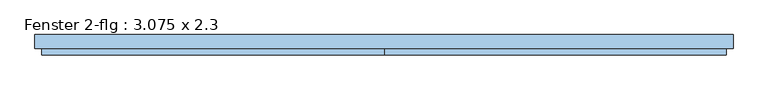
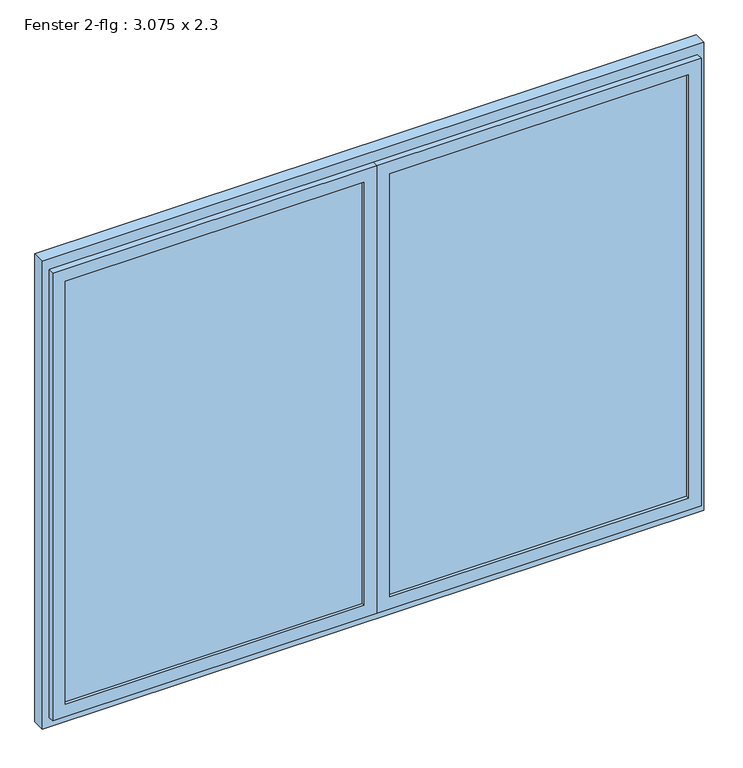
"""IFC4 building model written with IfcOpenShell, lengths in millimetres: window geometry, Fenster 2-flg : 3.075 x 2.3."""

from ifc_helpers import new_model, si_unit, frame, origin, place, context, project, spatial, polyline, outline, extrude, faceted_brep, source, transform, mapped, element, save


def fenster_2_flg_3_075_x_2_3_a01fdd74(model_context):
    return source(origin(), model_context, "Body", "SolidModel", [
        extrude(outline(polyline([(30.0, -30.0), (-30.0, -30.0), (-30.0, 30.0), (30.0, 30.0), (30.0, -30.0)])), frame((0.0, 0.0, 1080.0), z_axis=(0.0, 0.0, 1.0), x_axis=(1.0, 0.0, 0.0)), (0.0, 0.0, 1.0), 2140.0),
        extrude(outline(polyline([(3300.0, -1537.5), (1000.0, -1537.5), (1000.0, 1537.5), (3300.0, 1537.5), (3300.0, -1537.5)]), holes=[polyline([(3220.0, -1477.5), (3220.0, 1477.5), (1080.0, 1477.5), (1080.0, -1477.5), (3220.0, -1477.5)])]), frame((0.0, -30.0, 0.0), z_axis=(0.0, 1.0, 0.0), x_axis=(0.0, 0.0, 1.0)), (0.0, 0.0, 1.0), 60.0),
        faceted_brep([(-1477.5, -30.0, 1080.0), (-1477.5, 0.0, 1080.0), (-30.0, 0.0, 1080.0), (-30.0, -30.0, 1080.0), (-30.0, 0.0, 3220.0), (-30.0, -30.0, 3220.0), (-1477.5, 0.0, 3220.0), (-60.0, 0.0, 3190.0), (-1447.5, 0.0, 3190.0), (-1447.5, 0.0, 1110.0), (-60.0, 0.0, 1110.0), (0.0, -30.0, 1050.0), (-1507.5, -30.0, 1050.0), (-1507.5, -30.0, 3250.0), (0.0, -30.0, 3250.0), (-1477.5, -30.0, 3220.0), (-1507.5, -60.0, 1050.0), (0.0, -60.0, 1050.0), (0.0, -60.0, 3250.0), (-1507.5, -60.0, 3250.0), (-60.0, -60.0, 1110.0), (-1447.5, -60.0, 1110.0), (-1447.5, -60.0, 3190.0), (-60.0, -60.0, 3190.0)], [[[0, 1, 2, 3]], [[3, 2, 4, 5]], [[2, 1, 6, 4], [7, 8, 9, 10]], [[11, 12, 13, 14], [5, 15, 0, 3]], [[16, 12, 11, 17]], [[17, 11, 14, 18]], [[18, 19, 16, 17], [20, 21, 22, 23]], [[9, 21, 20, 10]], [[10, 20, 23, 7]], [[15, 6, 1, 0]], [[19, 13, 12, 16]], [[8, 22, 21, 9]], [[5, 4, 6, 15]], [[18, 14, 13, 19]], [[7, 23, 22, 8]]]),
        faceted_brep([(30.0, -30.0, 1080.0), (30.0, 0.0, 1080.0), (1477.5, 0.0, 1080.0), (1477.5, -30.0, 1080.0), (1477.5, 0.0, 3220.0), (1477.5, -30.0, 3220.0), (30.0, 0.0, 3220.0), (1447.5, 0.0, 3190.0), (60.0, 0.0, 3190.0), (60.0, 0.0, 1110.0), (1447.5, 0.0, 1110.0), (1507.5, -30.0, 1050.0), (0.0, -30.0, 1050.0), (0.0, -30.0, 3250.0), (1507.5, -30.0, 3250.0), (30.0, -30.0, 3220.0), (0.0, -60.0, 1050.0), (1507.5, -60.0, 1050.0), (1507.5, -60.0, 3250.0), (0.0, -60.0, 3250.0), (1447.5, -60.0, 1110.0), (60.0, -60.0, 1110.0), (60.0, -60.0, 3190.0), (1447.5, -60.0, 3190.0)], [[[0, 1, 2, 3]], [[3, 2, 4, 5]], [[2, 1, 6, 4], [7, 8, 9, 10]], [[11, 12, 13, 14], [5, 15, 0, 3]], [[16, 12, 11, 17]], [[17, 11, 14, 18]], [[18, 19, 16, 17], [20, 21, 22, 23]], [[9, 21, 20, 10]], [[10, 20, 23, 7]], [[15, 6, 1, 0]], [[19, 13, 12, 16]], [[8, 22, 21, 9]], [[5, 4, 6, 15]], [[18, 14, 13, 19]], [[7, 23, 22, 8]]]),
        extrude(outline(polyline([(60.0, -15.0), (1447.5, -15.0), (1447.5, -45.0), (60.0, -45.0), (60.0, -15.0)])), frame((0.0, 0.0, 1110.0), z_axis=(0.0, 0.0, 1.0), x_axis=(1.0, 0.0, 0.0)), (0.0, 0.0, 1.0), 2080.0),
        extrude(outline(polyline([(-1447.5, -15.0), (-60.0, -15.0), (-60.0, -45.0), (-1447.5, -45.0), (-1447.5, -15.0)])), frame((0.0, 0.0, 1110.0), z_axis=(0.0, 0.0, 1.0), x_axis=(1.0, 0.0, 0.0)), (0.0, 0.0, 1.0), 2080.0),
    ])


if __name__ == "__main__":
    model = new_model("IFC4")
    model_context = context("Model", 3, world=origin())
    ifc_project = project(units=[si_unit("LENGTHUNIT", "METRE", prefix="MILLI")], contexts=[model_context])
    site = spatial("IfcSite", under=ifc_project)
    building = spatial("IfcBuilding", under=site)
    placement = place(None, origin())
    fenster_2_flg_3_075_x_2_3_shape = fenster_2_flg_3_075_x_2_3_a01fdd74(model_context)
    element("IfcWindow", 1, ObjectType="Fenster 2-flg : 3.075 x 2.3", at=placement, inside=building, context=model_context, shape_type="MappedRepresentation", body=[
        mapped(fenster_2_flg_3_075_x_2_3_shape, transform((0.0, 0.0, 0.0), x_axis=(1.0, 0.0, 0.0), y_axis=(0.0, 1.0, 0.0), z_axis=(0.0, 0.0, 1.0))),
    ])
    save(model, "model.ifc")

# Revit data of these elements
# Type "Fenster 2-flg : 3.075 x 2.3"
#   Type Mark = "73"
#   Operation = "DoublePanelVertical"
#   Keynote = "16.05.01"
#   Visual Light Transmittance = 0.9
#   Solar Heat Gain Coefficient = 0.78
#   Rough Width = 3.075 m
#   Rough Height = 2.300 m
#   Heat Transfer Coefficient (U) = 3.6886 W/(m²·K)
#   Rahmentiefe = 0.060 m
#   Rahmenhöhe unten = 0.080 m
#   Höhe oberer  Rahmen = 0.080 m
#   Rahmenbreite = 0.060 m
#   Height = 2.300 m
#   Tiefe Flügel = 0.060 m
#   Flügelbreite = 0.060 m
#   Einbautiefe (von außen) [instance default] = 0.140 m
#   Width = 3.075 m
#   Öffnungsrichtung oben [instance default] = yes
#   Öffnungsrichtung in Draufsicht anzeigen [instance default] = no
#   Drehflügel 1 [instance default] = yes
#   Bild [instance default] = none
#   Glas [instance default] = none
#   Fensterflügel [instance default] = none
#   Äußere Fensterbank [instance default] = none
#   Innere Fensterbank [instance default] = none
#   Construction Type Id = ""
#   Wall Closure = (empty or 0)
#   Analytic Construction = (empty or 0)
# Element 1 (IfcWindow, "Fenster 2-flg : 3.075 x 2.3")
#   Einbautiefe (von außen) = 0.120 m
#   Materials on its faces: "Kunststoff - Weiß", "Glas"
# Materials
#   "Kunststoff - Weiß": class "Kunststoff", colour RGB 249 249 249, transparency 0, Cost = 0
#   "Glas": class "Glas", colour RGB 0 0 255, transparency 0.75, Comments = "Render-Darstellung nicht aktualisiert ", Cost = 0
